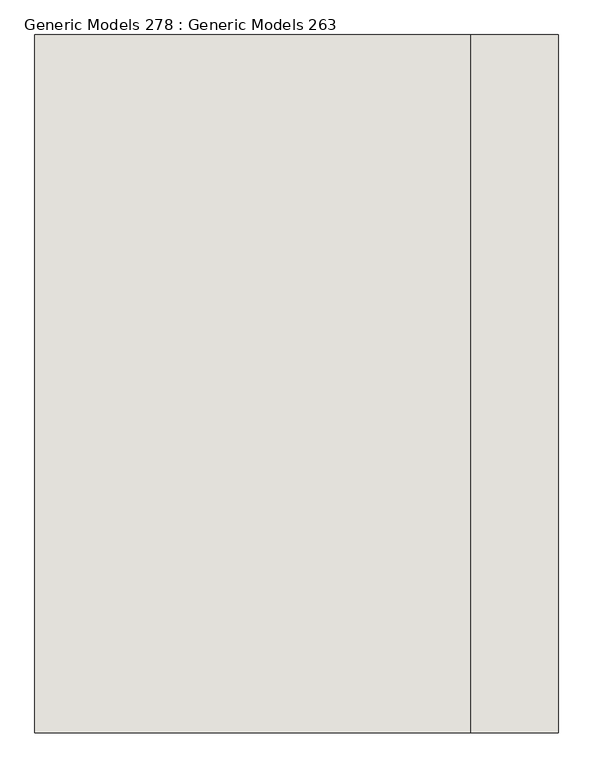
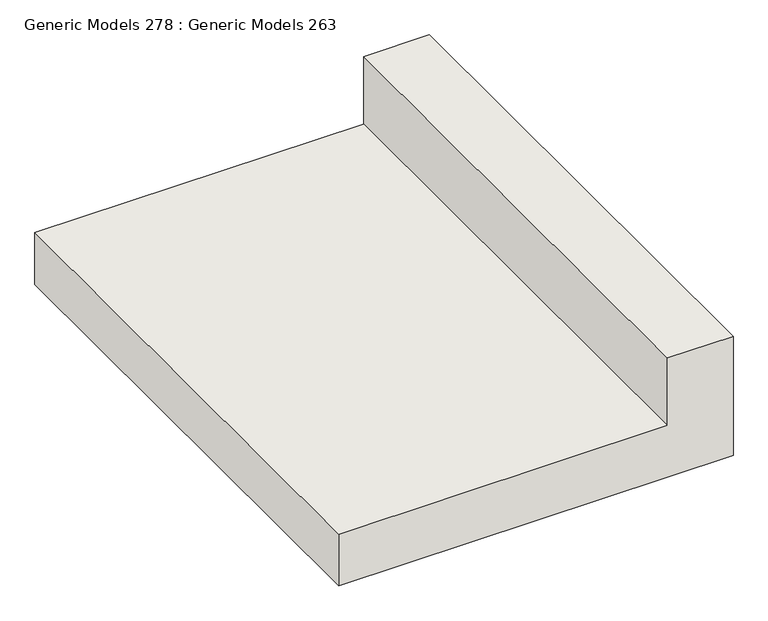
"""IFC4 building model written with IfcOpenShell, lengths in millimetres: wall geometry, Generic Models 278 : Generic Models 263."""

from ifc_helpers import new_model, si_unit, frame, origin, place, context, project, spatial, polyline, outline, extrude, source, transform, mapped, element, save


def generic_models_278_generic_models_263_5a7632f5(model_context):
    return source(origin(), model_context, "Body", "SweptSolid", [
        extrude(outline(polyline([(-381.0, 60947.5797726), (-381.0, 60185.5797726), (-508.0, 60185.5797726), (-508.0, 61099.9797726), (-215.9, 61099.9797726), (-215.9, 60947.5797726), (-381.0, 60947.5797726)])), frame((0.0, -94.4486541, 0.0), z_axis=(0.0, 1.0, 0.0), x_axis=(0.0, 0.0, 1.0)), (0.0, 0.0, 1.0), 1219.2),
    ])


if __name__ == "__main__":
    model = new_model("IFC4")
    model_context = context("Model", 3, world=origin())
    ifc_project = project(units=[si_unit("LENGTHUNIT", "METRE", prefix="MILLI")], contexts=[model_context])
    site = spatial("IfcSite", under=ifc_project)
    building = spatial("IfcBuilding", under=site)
    placement = place(None, origin())
    generic_models_278_generic_models_263_shape = generic_models_278_generic_models_263_5a7632f5(model_context)
    element("IfcWall", 1, ObjectType="Generic Models 278 : Generic Models 263", at=placement, inside=building, context=model_context, shape_type="MappedRepresentation", body=[
        mapped(generic_models_278_generic_models_263_shape, transform((0.0, 0.0, 0.0), x_axis=(1.0, 0.0, 0.0), y_axis=(0.0, 1.0, 0.0), z_axis=(0.0, 0.0, 1.0))),
    ])
    save(model, "model.ifc")

# Revit data of these elements
# Element 1 (IfcWall, "Generic Models 278 : Generic Models 263")
#   Materials on its faces: "5\" MIN. COMPACTED BASE AGGREGATE UNDER CURB"
# Materials
#   "5\" MIN. COMPACTED BASE AGGREGATE UNDER CURB": class "Miscellaneous", colour RGB 183 184 198, transparency 0, Cost = 0
